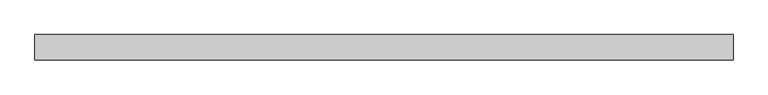
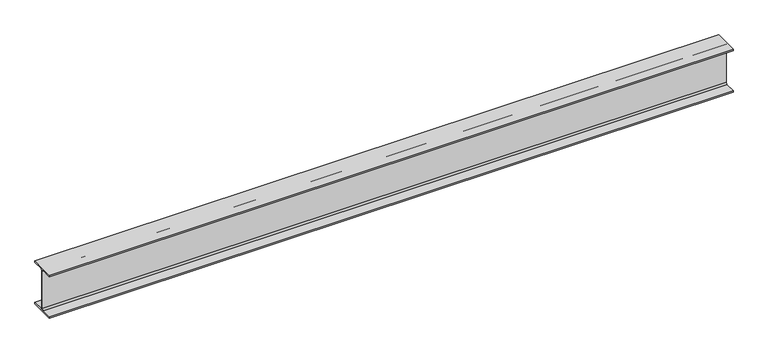
"""IFC4 building model written with IfcOpenShell, lengths in millimetres: beam geometry, Old_Steel Beam_H-KSD3502 : H_SB_ASB_H-250×125x6x9."""

from ifc_helpers import new_model, si_unit, point, frame, frame_2d, origin, place, context, project, spatial, polyline, circle_curve, trimmed, segment, composite_curve, outline, extrude, source, transform, mapped, element, save


def beam_eb6811aa(model_context):
    return source(origin(), model_context, "Body", "SweptSolid", [
        extrude(outline(composite_curve([segment(polyline([(82.5, -141.5), (82.5, -151.7), (-82.5, -151.7), (-82.5, -141.5), (-11.9, -141.5)]), True, "CONTINUOUS"), segment(trimmed(circle_curve(frame_2d((-11.9, -132.6)), 8.9), [point((-11.9, -141.5))], [point((-3.0, -132.6))], True, "CARTESIAN"), True, "CONTINUOUS"), segment(polyline([(-3.0, -132.6), (-3.0, 132.6)]), True, "CONTINUOUS"), segment(trimmed(circle_curve(frame_2d((-11.9, 132.6)), 8.9), [point((-3.0, 132.6))], [point((-11.9, 141.5))], True, "CARTESIAN"), True, "CONTINUOUS"), segment(polyline([(-11.9, 141.5), (-82.5, 141.5), (-82.5, 151.7), (82.5, 151.7), (82.5, 141.5), (11.9, 141.5)]), True, "CONTINUOUS"), segment(trimmed(circle_curve(frame_2d((11.9, 132.6)), 8.9), [point((11.9, 141.5))], [point((3.0, 132.6))], True, "CARTESIAN"), True, "CONTINUOUS"), segment(polyline([(3.0, 132.6), (3.0, -132.6)]), True, "CONTINUOUS"), segment(trimmed(circle_curve(frame_2d((11.9, -132.6)), 8.9), [point((3.0, -132.6))], [point((11.9, -141.5))], True, "CARTESIAN"), True, "CONTINUOUS"), segment(polyline([(11.9, -141.5), (82.5, -141.5)]), True, "CONTINUOUS")], self_intersect=False)), frame((-2404.8, 0.0, 0.0), z_axis=(1.0, 0.0, 0.0), x_axis=(0.0, 1.0, 0.0)), (0.0, 0.0, 1.0), 4569.2729123),
    ])


if __name__ == "__main__":
    model = new_model("IFC4")
    model_context = context("Model", 3, world=origin())
    ifc_project = project(units=[si_unit("LENGTHUNIT", "METRE", prefix="MILLI")], contexts=[model_context])
    site = spatial("IfcSite", under=ifc_project)
    building = spatial("IfcBuilding", under=site)
    placement = place(None, origin())
    beam_shape = beam_eb6811aa(model_context)
    element("IfcBeam", 1, ObjectType="Old_Steel Beam_H-KSD3502 : H_SB_ASB_H-250×125x6x9", at=placement, inside=building, context=model_context, shape_type="MappedRepresentation", body=[
        mapped(beam_shape, transform((0.0, 0.0, 0.0), x_axis=(1.0, 0.0, 0.0), y_axis=(0.0, 1.0, 0.0), z_axis=(0.0, 0.0, 1.0))),
    ])
    save(model, "model.ifc")

# Revit data of these elements
# Type "Old_Steel Beam_H-KSD3502 : H_SB_ASB_H-250×125x6x9"
#   Width = 12.5 cm
#   Web Thickness = 0.6 cm
#   Web Fillet = 1.2 cm
#   Warping Constant = 42539.8 cm⁶
#   Torsional Moment of Inertia = 7.8102 cm⁴
#   Torsional Modulus = 1.0 cm³
#   Section Area = 37.66 cm²
#   Plastic Modulus weak axis = 73.1 cm³
#   Plastic Modulus strong axis = 366.0 cm³
#   Perimeter = 0.97 m²/m
#   Nominal Weight = 29.60 kgf/m
#   Moment of Inertia weak axis = 294.00 cm⁴
#   Moment of Inertia strong axis = 4050.00 cm⁴
#   Height = 25.0 cm
#   Flange Thickness = 0.9 cm
#   Elastic Modulus weak axis = 47.0 cm³
#   Elastic Modulus strong axis = 324.0 cm³
#   Centroid Vertical = 12.5 cm
#   Centroid Horizontal = 6.25 cm
#   Length [instance default] = 1.5240 m
#   Structural Material [instance default] = Steel, 45-345
#   Assembly Code = ""
# Element 1 (IfcBeam, "Old_Steel Beam_H-KSD3502 : H_SB_ASB_H-250×125x6x9")
#   Structural Material = none
# Materials
#   "Steel, 45-345": class "Metal", colour RGB 189 187 185, transparency 0, Description = "Steel 345 MPa", Cost = 0
